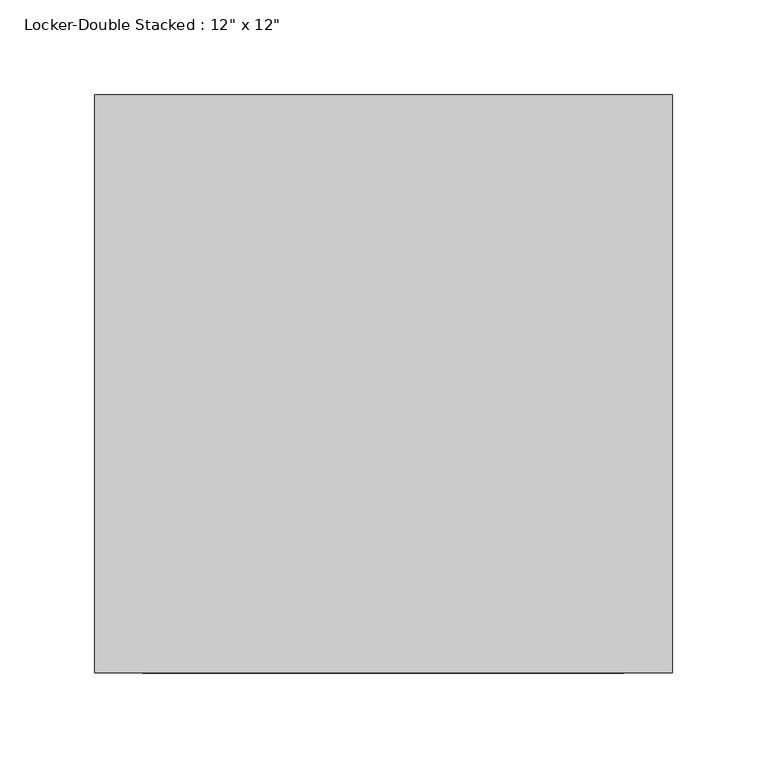
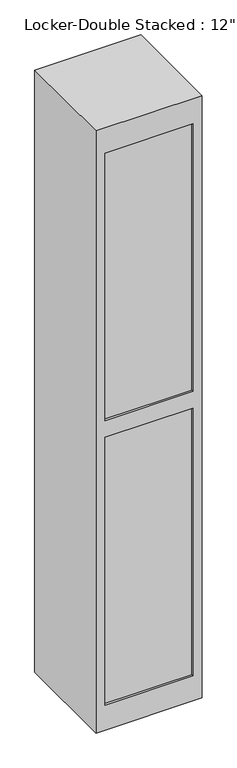
"""IFC4 building model written with IfcOpenShell, lengths in millimetres: furniture geometry."""

from ifc_helpers import new_model, si_unit, origin, place, context, project, spatial, faceted_brep, source, transform, mapped, element, save


def furniture_200c970f(model_context):
    return source(origin(), model_context, "Body", "Brep", [
        faceted_brep([(152.4, -152.4, 1828.8), (152.4, 152.4, 1828.8), (-152.4, 152.4, 1828.8), (-152.4, -152.4, 1828.8), (152.4, -152.4, 0.0), (-152.4, -152.4, 0.0), (-152.4, 152.4, 0.0), (152.4, 152.4, 0.0), (127.0, -152.4, 889.0), (127.0, -152.4, 76.2), (-127.0, -152.4, 76.2), (-127.0, -152.4, 889.0), (-127.0, -152.4, 1752.6), (127.0, -152.4, 1752.6), (127.0, -152.4, 939.8), (-127.0, -152.4, 939.8), (127.0, -146.05, 76.2), (127.0, -146.05, 889.0), (-127.0, -146.05, 889.0), (-127.0, -146.05, 76.2), (127.0, -146.05, 1752.6), (-127.0, -146.05, 1752.6), (-127.0, -146.05, 939.8), (127.0, -146.05, 939.8)], [[[0, 1, 2, 3]], [[4, 5, 6, 7]], [[1, 0, 4, 7]], [[2, 1, 7, 6]], [[3, 2, 6, 5]], [[0, 3, 5, 4], [8, 9, 10, 11], [12, 13, 14, 15]], [[16, 17, 18, 19]], [[17, 16, 9, 8]], [[18, 17, 8, 11]], [[19, 18, 11, 10]], [[16, 19, 10, 9]], [[20, 21, 22, 23]], [[21, 20, 13, 12]], [[22, 21, 12, 15]], [[23, 22, 15, 14]], [[20, 23, 14, 13]]]),
    ])


if __name__ == "__main__":
    model = new_model("IFC4")
    model_context = context("Model", 3, world=origin())
    ifc_project = project(units=[si_unit("LENGTHUNIT", "METRE", prefix="MILLI")], contexts=[model_context])
    site = spatial("IfcSite", under=ifc_project)
    building = spatial("IfcBuilding", under=site)
    placement = place(None, origin())
    furniture_shape = furniture_200c970f(model_context)
    element("IfcFurniture", 1, ObjectType="Locker-Double Stacked : 12\" x 12\"", at=placement, inside=building, context=model_context, shape_type="MappedRepresentation", body=[
        mapped(furniture_shape, transform((0.0, 0.0, 0.0), x_axis=(1.0, 0.0, 0.0), y_axis=(0.0, 1.0, 0.0), z_axis=(0.0, 0.0, 1.0))),
    ])
    save(model, "model.ifc")

# Revit data of these elements
# Type "Locker-Double Stacked : 12\" x 12\""
#   Assembly Code = "E2010"
#   Depth = 1' - 0"
#   Height = 6' - 0"
#   Width = 1' - 0"
#   Material = Metal - Paint Finish - Dark Gray, Matte
# Element 1 (IfcFurniture, "Locker-Double Stacked : 12\" x 12\"")
#   Materials on its faces: "Metal - Paint Finish - Dark Gray, Matte"
# Materials
#   "Metal - Paint Finish - Dark Gray, Matte": class "Metal", colour RGB 98 98 98, transparency 0
